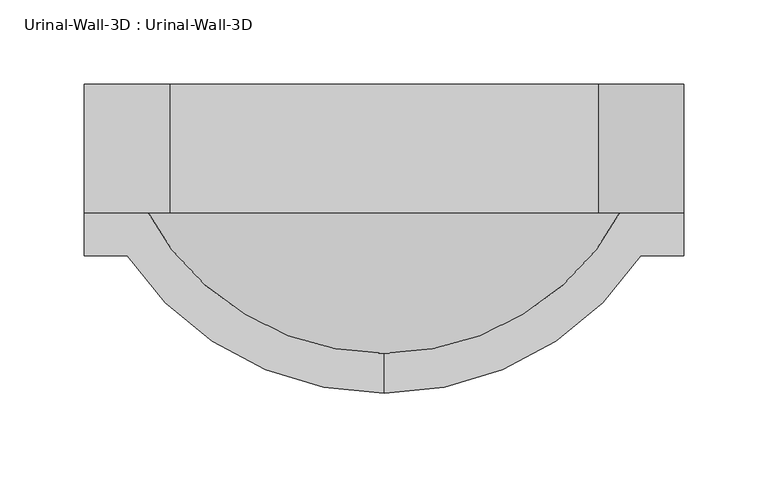
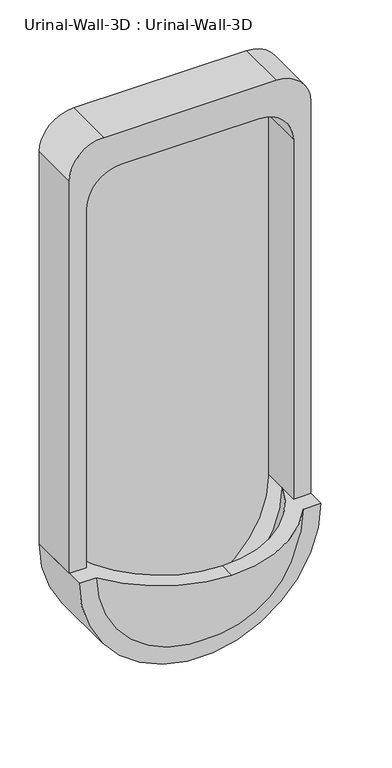
"""IFC4 building model written with IfcOpenShell, lengths in millimetres: flow terminal geometry, Urinal-Wall-3D : Urinal-Wall-3D."""

from ifc_helpers import new_model, si_unit, point, frame, frame_2d, origin, place, context, project, spatial, polyline, circle_curve, ellipse_curve, trimmed, segment, composite_curve, outline, extrude, source, transform, mapped, element, save
from ifc_brep_helpers import plane_surface, cylinder_surface, revolved_surface, advanced_brep


def urinal_wall_3d_urinal_wall_3d_87f6c982(model_context):
    return source(origin(), model_context, "Body", "SolidModel", [
        extrude(outline(composite_curve([segment(polyline([(609.6, 43.3254001), (609.6, 68.7254001), (1219.2, 68.7254001)]), True, "CONTINUOUS"), segment(trimmed(circle_curve(frame_2d((1219.2, 17.9254001)), 50.8), [point((1219.2, 68.7254001))], [point((1270.0, 17.9254001))], False, "CARTESIAN"), True, "CONTINUOUS"), segment(polyline([(1270.0, 17.9254001), (1270.0, -236.0745999)]), True, "CONTINUOUS"), segment(trimmed(circle_curve(frame_2d((1219.2, -236.0745999)), 50.8), [point((1270.0, -236.0745999))], [point((1219.2, -286.8745999))], False, "CARTESIAN"), True, "CONTINUOUS"), segment(polyline([(1219.2, -286.8745999), (609.6, -286.8745999), (609.6, -261.4745999), (1168.4, -261.4745999)]), True, "CONTINUOUS"), segment(trimmed(circle_curve(frame_2d((1168.4, -210.6745999)), 50.8), [point((1168.4, -261.4745999))], [point((1219.2, -210.6745999))], True, "CARTESIAN"), True, "CONTINUOUS"), segment(polyline([(1219.2, -210.6745999), (1219.2, -7.4745999)]), True, "CONTINUOUS"), segment(trimmed(circle_curve(frame_2d((1168.4, -7.4745999)), 50.8), [point((1219.2, -7.4745999))], [point((1168.4, 43.3254001))], True, "CARTESIAN"), True, "CONTINUOUS"), segment(polyline([(1168.4, 43.3254001), (609.6, 43.3254001)]), True, "CONTINUOUS")], self_intersect=False)), frame((0.0, -274.6375, 0.0), z_axis=(0.0, 1.0, 0.0), x_axis=(0.0, 0.0, 1.0)), (0.0, 0.0, 1.0), 76.2),
        extrude(outline(composite_curve([segment(trimmed(circle_curve(frame_2d((1168.4, -7.4745999)), 50.8), [point((1168.4, 43.3254001))], [point((1219.2, -7.4745999))], False, "CARTESIAN"), True, "CONTINUOUS"), segment(polyline([(1219.2, -7.4745999), (1219.2, -210.6745999)]), True, "CONTINUOUS"), segment(trimmed(circle_curve(frame_2d((1168.4, -210.6745999)), 50.8), [point((1219.2, -210.6745999))], [point((1168.4, -261.4745999))], False, "CARTESIAN"), True, "CONTINUOUS"), segment(polyline([(1168.4, -261.4745999), (609.6, -261.4745999)]), True, "CONTINUOUS"), segment(trimmed(circle_curve(frame_2d((609.6, -109.0745999)), 152.4), [point((609.6, -261.4745999))], [point((609.6, 43.3254001))], False, "CARTESIAN"), True, "CONTINUOUS"), segment(polyline([(609.6, 43.3254001), (1168.4, 43.3254001)]), True, "CONTINUOUS")], self_intersect=False)), frame((0.0, -211.1375, 0.0), z_axis=(0.0, 1.0, 0.0), x_axis=(0.0, 0.0, 1.0)), (0.0, 0.0, 1.0), 12.7),
        advanced_brep(
        [(-109.0745999, -381.5995048, 609.6), (43.3254001, -300.0375, 609.6), (68.7254001, -300.0375, 609.6), (68.7254001, -198.4375, 609.6), (43.3254001, -198.4375, 609.6), (43.3254001, -245.3081063, 609.6), (-109.0745999, -357.8822043, 609.6), (-261.4745999, -245.3081063, 609.6), (-261.4745999, -198.4375, 609.6), (-286.8745999, -198.4375, 609.6), (-286.8745999, -300.0375, 609.6), (-261.4745999, -300.0375, 609.6)],
        [
            (0, 1, circle_curve(frame((-109.0745999, -198.4375, 609.6), z_axis=(0.0, 0.0, 1.0), x_axis=(1.0, 0.0, 0.0)), 183.1620048)),
            (1, 2),
            (2, 3),
            (3, 4),
            (4, 5),
            (5, 6, circle_curve(frame((-109.0745999, -198.4375, 609.6), z_axis=(0.0, 0.0, -1.0), x_axis=(1.0, 0.0, 0.0)), 159.4447043)),
            (6, 0),
            (6, 7, circle_curve(frame((-109.0745999, -198.4375, 609.6), z_axis=(0.0, 0.0, -1.0), x_axis=(-1.0, 0.0, 0.0)), 159.4447043)),
            (7, 8),
            (8, 9),
            (9, 10),
            (10, 11),
            (11, 0, circle_curve(frame((-109.0745999, -198.4375, 609.6), z_axis=(0.0, 0.0, 1.0), x_axis=(-1.0, 0.0, 0.0)), 183.1620048)),
            (5, 7, circle_curve(frame((-109.0745999, -245.3081063, 609.6), z_axis=(0.0, 1.0, 0.0), x_axis=(1.0, 0.0, 0.0)), 152.4)),
            (4, 8, circle_curve(frame((-109.0745999, -198.4375, 609.6), z_axis=(0.0, 1.0, 0.0), x_axis=(1.0, 0.0, 0.0)), 152.4)),
            (3, 9, circle_curve(frame((-109.0745999, -198.4375, 609.6), z_axis=(0.0, 1.0, 0.0), x_axis=(1.0, 0.0, 0.0)), 177.8)),
            (2, 10, circle_curve(frame((-109.0745999, -300.0375, 609.6), z_axis=(0.0, 1.0, 0.0), x_axis=(1.0, 0.0, 0.0)), 177.8)),
            (1, 11, circle_curve(frame((-109.0745999, -300.0375, 609.6), z_axis=(0.0, 1.0, 0.0), x_axis=(1.0, 0.0, 0.0)), 152.4)),
        ],
        [
            plane_surface(frame((-109.0745999, -487.6479173, 609.6), z_axis=(0.0, 0.0, 1.0), x_axis=(1.0, 0.0, 0.0))),
            plane_surface(frame((-109.0745999, -487.6479173, 609.6), z_axis=(0.0, 0.0, 1.0), x_axis=(-1.0, 0.0, 0.0))),
            revolved_surface(trimmed(ellipse_curve(frame((-109.0745999, -198.4375, 609.6), z_axis=(0.0, 0.0, 1.0), x_axis=(1.0, 0.0, 0.0)), 159.4447043, 159.4447043), [point((-109.0745999, -357.8822043, 609.6))], [point((43.3254001, -245.3081063, 609.6))], True, "CARTESIAN"), (-109.0745999, -487.6479173, 609.6), (0.0, -1.0, 0.0)),
            revolved_surface(polyline([(43.32540010000001, -245.3081063, 609.6), (43.32540010000001, -198.4375, 609.6)]), (-109.0745999, -487.6479173, 609.6), (0.0, -1.0, 0.0)),
            plane_surface(frame((-109.0745999, -198.4375, 609.6), z_axis=(0.0, 1.0, 0.0), x_axis=(1.0, 0.0, 0.0))),
            cylinder_surface(frame((-109.0745999, -487.6479173, 609.6), z_axis=(0.0, -1.0, 0.0), x_axis=(1.0, 0.0, 0.0)), 177.8),
            plane_surface(frame((-109.0745999, -300.0375, 609.6), z_axis=(0.0, -1.0, 0.0), x_axis=(1.0, 0.0, 0.0))),
            revolved_surface(trimmed(ellipse_curve(frame((-109.0745999, -198.4375, 609.6), z_axis=(0.0, 0.0, -1.0), x_axis=(1.0, 0.0, 0.0)), 183.1620048, 183.1620048), [point((43.3254001, -300.0375, 609.6))], [point((-109.0745999, -381.5995048, 609.6))], True, "CARTESIAN"), (-109.0745999, -487.6479173, 609.6), (0.0, -1.0, 0.0)),
        ],
        [
            (0, [[1, 2, 3, 4, 5, 6, 7]]),
            (1, [[-7, 8, 9, 10, 11, 12, 13]]),
            (2, [[-8, -6, 14]]),
            (3, [[-9, -14, -5, 15]]),
            (4, [[-10, -15, -4, 16]]),
            (5, [[-11, -16, -3, 17]]),
            (6, [[-12, -17, -2, 18]]),
            (7, [[-13, -18, -1]]),
        ],
    ),
    ])


if __name__ == "__main__":
    model = new_model("IFC4")
    model_context = context("Model", 3, world=origin())
    ifc_project = project(units=[si_unit("LENGTHUNIT", "METRE", prefix="MILLI")], contexts=[model_context])
    site = spatial("IfcSite", under=ifc_project)
    building = spatial("IfcBuilding", under=site)
    placement = place(None, origin())
    urinal_wall_3d_urinal_wall_3d_shape = urinal_wall_3d_urinal_wall_3d_87f6c982(model_context)
    element("IfcFlowTerminal", 1, ObjectType="Urinal-Wall-3D : Urinal-Wall-3D", at=placement, inside=building, context=model_context, shape_type="MappedRepresentation", body=[
        mapped(urinal_wall_3d_urinal_wall_3d_shape, transform((0.0, 0.0, 0.0), x_axis=(1.0, 0.0, 0.0), y_axis=(0.0, 1.0, 0.0), z_axis=(0.0, 0.0, 1.0))),
    ])
    save(model, "model.ifc")

# Revit data of these elements
# Type "Urinal-Wall-3D : Urinal-Wall-3D"
#   Assembly Code = "D2010210"
#   Bowl Height = 2' - 0"
#   Urinal Material = Porcelain - Ivory
#   Default Elevation = 0
# Materials
#   "Porcelain - Ivory": class "Unassigned", colour RGB 247 247 239, transparency 0
